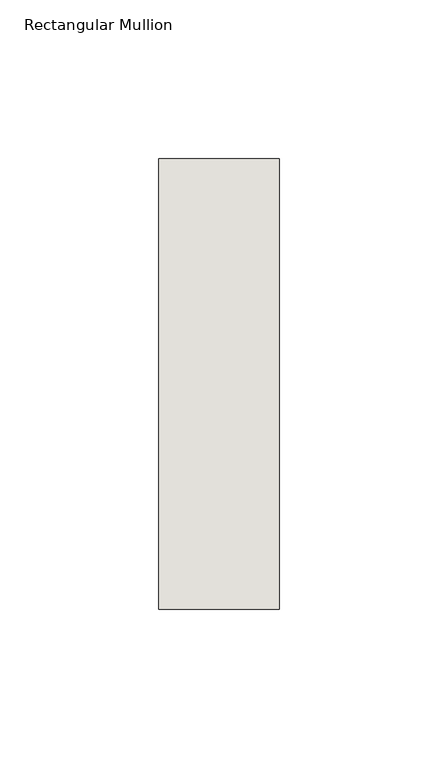
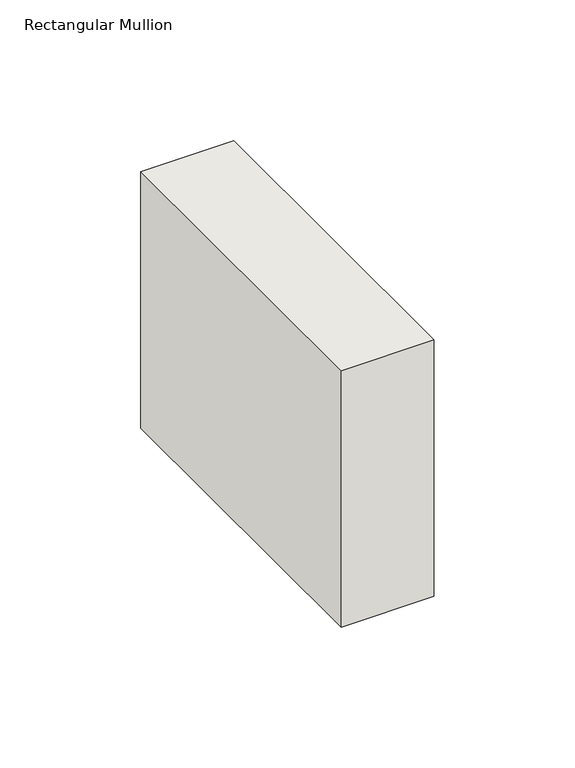
"""IFC4 building model written with IfcOpenShell, lengths in millimetres: wall geometry, Rectangular Mullion : NLRS_21_CWM_hsb-regel 38x142_gen_rsf."""

import ifcopenshell
import ifcopenshell.guid

model = None  # the IFC model being written
_history = None  # IfcOwnerHistory: only IFC2X3 demands one
_inside = {}  # id of a spatial element -> (the spatial element, [elements in it])
_under = {}  # id of a project, library or spatial element -> (it, [spatial elements below it])
_declared = {}  # id of a project -> (the project, [libraries it declares])
_typed = {}  # id of a type object -> (the type object, [elements of that type])
_made_of = {}  # id of a material, layer set ... -> (it, [elements and type objects made of it])


def new_model(schema):
    """Start an empty IFC model of exactly this schema.

    Asked for "IFC4X3", IfcOpenShell would pick the latest addendum, in which some entities
    have other attributes; the version numbers below select the first issue.
    IFC2X3 requires an IfcOwnerHistory on every rooted entity: one is made here for all.
    """
    global model, _history
    if schema == "IFC4X3":
        model = ifcopenshell.file(schema_version=(4, 3, 0, 0))
    else:
        model = ifcopenshell.file(schema=schema)
    _inside.clear()
    _under.clear()
    _declared.clear()
    _typed.clear()
    _made_of.clear()
    _history = None
    if model.schema == "IFC2X3":
        org = make("IfcOrganization", Name="unknown")
        user = make(
            "IfcPersonAndOrganization",
            ThePerson=make("IfcPerson", FamilyName="unknown"),
            TheOrganization=org,
        )
        app = make(
            "IfcApplication",
            ApplicationDeveloper=org,
            Version="unknown",
            ApplicationFullName="unknown",
            ApplicationIdentifier="unknown",
        )
        _history = make(
            "IfcOwnerHistory",
            OwningUser=user,
            OwningApplication=app,
            ChangeAction="ADDED",
            CreationDate=0,
        )
    return model


def make(cls, **values):
    """One entity of the class cls with the attributes given. An attribute that is None is left unset."""
    return model.create_entity(
        cls, **{name: value for name, value in values.items() if value is not None}
    )


def rooted(cls, **values):
    """An entity with a GlobalId (a new one), such as an element, a storey or a relation."""
    return make(cls, GlobalId=ifcopenshell.guid.new(), OwnerHistory=_history, **values)


def si_unit(unit_type, name, prefix=None):
    """IfcSIUnit, for example si_unit("LENGTHUNIT", "METRE", prefix="MILLI")."""
    return make("IfcSIUnit", UnitType=unit_type, Prefix=prefix, Name=name)


def assignment(units):
    """IfcUnitAssignment: the units of a project."""
    return None if units is None else make("IfcUnitAssignment", Units=units)


def point(xyz):
    """IfcCartesianPoint."""
    return None if xyz is None else make("IfcCartesianPoint", Coordinates=xyz)


def direction(xyz):
    """IfcDirection."""
    return None if xyz is None else make("IfcDirection", DirectionRatios=xyz)


def frame(location, z_axis=None, x_axis=None):
    """IfcAxis2Placement3D, a coordinate frame: its origin and axes. An axis left out is left unset."""
    return make(
        "IfcAxis2Placement3D",
        Location=point(location),
        Axis=direction(z_axis),
        RefDirection=direction(x_axis),
    )


def origin():
    """The frame at (0, 0, 0) with its axes left unset."""
    return frame((0.0, 0.0, 0.0))


def place(relative_to, where):
    """IfcLocalPlacement: puts the frame where relative to a parent placement (None: the world)."""
    return make(
        "IfcLocalPlacement", PlacementRelTo=relative_to, RelativePlacement=where
    )


def context(
    kind, dimensions, precision=None, world=None, true_north=None, identifier=None
):
    """IfcGeometricRepresentationContext, for example the 3D "Model" context."""
    return make(
        "IfcGeometricRepresentationContext",
        ContextIdentifier=identifier,
        ContextType=kind,
        CoordinateSpaceDimension=dimensions,
        Precision=precision,
        WorldCoordinateSystem=world,
        TrueNorth=true_north,
    )


def project(units=None, contexts=None):
    """IfcProject with its units and contexts."""
    return rooted(
        "IfcProject",
        Name="project",
        RepresentationContexts=contexts,
        UnitsInContext=assignment(units),
    )


def spatial(cls, under=None, at=None, **own):
    """A site, building, storey or space (cls), placed at a placement, below another one or the project."""
    s = rooted(cls, ObjectPlacement=at, **own)
    if under is not None:
        _under.setdefault(under.id(), (under, []))[1].append(s)
    return s


def polyline(points):
    """IfcPolyline through the points."""
    return make("IfcPolyline", Points=[point(p) for p in points])


def outline(outer, holes=None, kind="AREA"):
    """IfcArbitraryClosedProfileDef: a profile drawn as a closed curve; with holes, ...WithVoids."""
    if holes is None:
        return make("IfcArbitraryClosedProfileDef", ProfileType=kind, OuterCurve=outer)
    return make(
        "IfcArbitraryProfileDefWithVoids",
        ProfileType=kind,
        OuterCurve=outer,
        InnerCurves=holes,
    )


def extrude(swept, where, along, depth):
    """IfcExtrudedAreaSolid: the profile swept, set in the frame where, extruded along a direction by depth."""
    return make(
        "IfcExtrudedAreaSolid",
        SweptArea=swept,
        Position=where,
        ExtrudedDirection=direction(along),
        Depth=depth,
    )


def shape(context_of_items, identifier, shape_type, items):
    """IfcShapeRepresentation: the items that make up one representation, for example the "Body"."""
    return make(
        "IfcShapeRepresentation",
        ContextOfItems=context_of_items,
        RepresentationIdentifier=identifier,
        RepresentationType=shape_type,
        Items=items,
    )


def source(mapping_origin, context_of_items, identifier, shape_type, items):
    """IfcRepresentationMap: a shape defined once, which mapped items show again and again."""
    return make(
        "IfcRepresentationMap",
        MappingOrigin=mapping_origin,
        MappedRepresentation=shape(context_of_items, identifier, shape_type, items),
    )


def transform(
    local_origin,
    x_axis=None,
    y_axis=None,
    z_axis=None,
    scale=None,
    scale2=None,
    scale3=None,
    uniform=True,
):
    """IfcCartesianTransformationOperator3D, or its non-uniform kind. x_axis, y_axis, z_axis: its Axis1, 2, 3."""
    if uniform:
        return make(
            "IfcCartesianTransformationOperator3D",
            Axis1=direction(x_axis),
            Axis2=direction(y_axis),
            LocalOrigin=point(local_origin),
            Scale=scale,
            Axis3=direction(z_axis),
        )
    return make(
        "IfcCartesianTransformationOperator3DnonUniform",
        Axis1=direction(x_axis),
        Axis2=direction(y_axis),
        LocalOrigin=point(local_origin),
        Scale=scale,
        Axis3=direction(z_axis),
        Scale2=scale2,
        Scale3=scale3,
    )


def mapped(mapping_source, mapping_target):
    """IfcMappedItem: shows the shape of a source again, moved by a transform."""
    return make(
        "IfcMappedItem", MappingSource=mapping_source, MappingTarget=mapping_target
    )


def made_of(thing, what):
    """Note that an element or type object is made of a material, layer set ...; save() writes the relation."""
    if what is not None:
        _made_of.setdefault(what.id(), (what, []))[1].append(thing)
    return thing


def element(
    cls,
    number,
    at=None,
    inside=None,
    cuts=None,
    type_object=None,
    material=None,
    context=None,
    identifier="Body",
    shape_type=None,
    held_by="IfcProductDefinitionShape",
    body=None,
    shapes=None,
    **own,
):
    """One element of the class cls, such as IfcWall. Its Tag is "e" and its number.

    at: its placement. inside: the storey or other place that contains it. cuts: it is an
    opening in that element (IfcRelVoidsElement). A single representation is given by context,
    identifier, shape_type and body (its items); several are given by shapes. held_by: the class
    of the entity that holds the representations. save() writes the other relations.
    """
    e = rooted(cls, Tag="e%d" % number, ObjectPlacement=at, **own)
    if body is not None:
        shapes = [shape(context, identifier, shape_type, body)]
    if shapes is not None:
        e.Representation = make(held_by, Representations=shapes)
    if inside is not None:
        _inside.setdefault(inside.id(), (inside, []))[1].append(e)
    if cuts is not None:
        rooted(
            "IfcRelVoidsElement", RelatingBuildingElement=cuts, RelatedOpeningElement=e
        )
    if type_object is not None:
        _typed.setdefault(type_object.id(), (type_object, []))[1].append(e)
    return made_of(e, material)


def aggregate(whole, parts):
    """IfcRelAggregates: a whole, such as a stair, and the parts it consists of."""
    return rooted("IfcRelAggregates", RelatingObject=whole, RelatedObjects=parts)


def save(model, path):
    """Write the relations noted so far, then the file.

    IfcRelAggregates (storeys below a building ...), IfcRelContainedInSpatialStructure (elements
    in a storey), IfcRelDefinesByType, IfcRelAssociatesMaterial and IfcRelDeclares: one each for
    every whole, place, type object, material and project.
    """
    for whole, parts in _under.values():
        aggregate(whole, parts)
    for where, things in _inside.values():
        rooted(
            "IfcRelContainedInSpatialStructure",
            RelatedElements=things,
            RelatingStructure=where,
        )
    for kind, things in _typed.values():
        rooted("IfcRelDefinesByType", RelatedObjects=things, RelatingType=kind)
    for what, things in _made_of.values():
        rooted("IfcRelAssociatesMaterial", RelatedObjects=things, RelatingMaterial=what)
    for by, libraries in _declared.values():
        rooted("IfcRelDeclares", RelatingContext=by, RelatedDefinitions=libraries)
    model.write(path)


def rectangular_mullion_3ccaa2f0(model_context):
    return source(origin(), model_context, "Body", "SweptSolid", [
        extrude(outline(polyline([(-38.0, -71.0), (-38.0, 71.0), (0.0, 71.0), (0.0, -71.0), (-38.0, -71.0)])), frame((0.0, 0.0, -111.0), z_axis=(0.0, 0.0, 1.0), x_axis=(1.0, 0.0, 0.0)), (0.0, 0.0, 1.0), 111.0),
    ])


if __name__ == "__main__":
    model = new_model("IFC4")
    model_context = context("Model", 3, world=origin())
    ifc_project = project(units=[si_unit("LENGTHUNIT", "METRE", prefix="MILLI")], contexts=[model_context])
    site = spatial("IfcSite", under=ifc_project)
    building = spatial("IfcBuilding", under=site)
    placement = place(None, origin())
    rectangular_mullion_shape = rectangular_mullion_3ccaa2f0(model_context)
    element("IfcWall", 1, ObjectType="Rectangular Mullion : NLRS_21_CWM_hsb-regel 38x142_gen_rsf", at=placement, inside=building, context=model_context, shape_type="MappedRepresentation", body=[
        mapped(rectangular_mullion_shape, transform((0.0, 0.0, 0.0), x_axis=(1.0, 0.0, 0.0), y_axis=(0.0, 1.0, 0.0), z_axis=(0.0, 0.0, 1.0))),
    ])
    save(model, "model.ifc")

# Revit data of these elements
# Type "Rectangular Mullion : NLRS_21_CWM_hsb-regel 38x142_gen_rsf"
#   Type IfcGUID = "07M7mRoiH1CR8m_RSKIwpF"
#   Assembly Code = "21.10"
#   IfcExportAs = "IfcWall"
#   built-in parameter 1007322 = 0.465879 (stored number, unit not read)
#   built-in parameter 1007321 = 0.062336 (stored number, unit not read)
#   built-in parameter 1007320 = 0.062336 (stored number, unit not read)
# Element 1 (IfcWall, "Rectangular Mullion : NLRS_21_CWM_hsb-regel 38x142_gen_rsf")
#   Materials on its faces: "NLRS_i2_hout naaldhout vuren_gen_rsf"
# Materials
#   "NLRS_i2_hout naaldhout vuren_gen_rsf": class "I - Hout", colour RGB 234 199 147, transparency 0, Keynote = "i2", Manufacturer = "Revit Standards Foundation", URL = "www.revitstandards.org", Description = "hout vuren", Cost = 0
